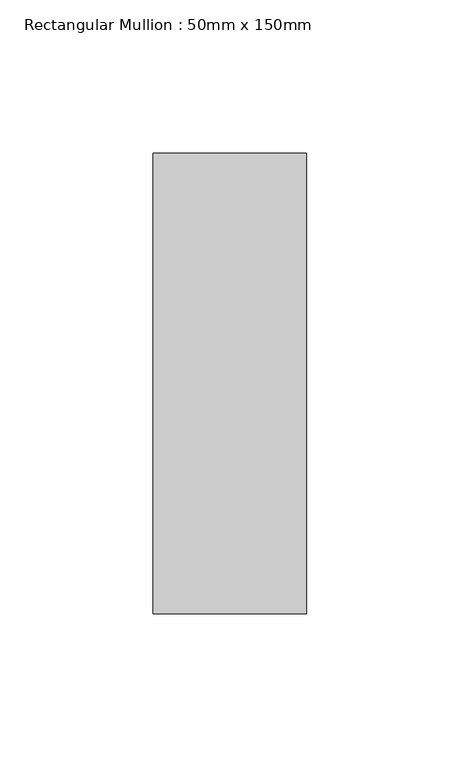
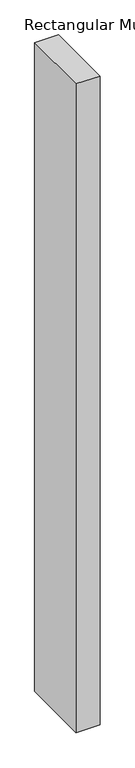
"""IFC4 building model written with IfcOpenShell, lengths in millimetres: member geometry, Rectangular Mullion : 50mm x 150mm."""

from ifc_helpers import new_model, si_unit, frame, origin, place, context, project, spatial, polyline, outline, extrude, source, transform, mapped, element, save


def rectangular_mullion_50mm_x_150mm_f5d81ac7(model_context):
    return source(origin(), model_context, "Body", "SweptSolid", [
        extrude(outline(polyline([(0.0, 75.0), (0.0, -75.0), (-50.0, -75.0), (-50.0, 75.0), (0.0, 75.0)])), frame((0.0, 0.0, -1436.0169252), z_axis=(0.0, 0.0, 1.0), x_axis=(1.0, 0.0, 0.0)), (0.0, 0.0, 1.0), 1436.0169252),
    ])


if __name__ == "__main__":
    model = new_model("IFC4")
    model_context = context("Model", 3, world=origin())
    ifc_project = project(units=[si_unit("LENGTHUNIT", "METRE", prefix="MILLI")], contexts=[model_context])
    site = spatial("IfcSite", under=ifc_project)
    building = spatial("IfcBuilding", under=site)
    placement = place(None, origin())
    rectangular_mullion_50mm_x_150mm_shape = rectangular_mullion_50mm_x_150mm_f5d81ac7(model_context)
    element("IfcMember", 1, ObjectType="Rectangular Mullion : 50mm x 150mm", at=placement, inside=building, context=model_context, shape_type="MappedRepresentation", body=[
        mapped(rectangular_mullion_50mm_x_150mm_shape, transform((0.0, 0.0, 0.0), x_axis=(1.0, 0.0, 0.0), y_axis=(0.0, 1.0, 0.0), z_axis=(0.0, 0.0, 1.0))),
    ])
    save(model, "model.ifc")

# Revit data of these elements
# Type "Rectangular Mullion : 50mm x 150mm"
#   built-in parameter 1007304 = 0.492126 (stored number, unit not read)
#   built-in parameter 1007301 = 0.082021 (stored number, unit not read)
#   built-in parameter 1007300 = 0.082021 (stored number, unit not read)
# Element 1 (IfcMember, "Rectangular Mullion : 50mm x 150mm")
#   Materials on its faces: "Aluminum"
# Materials
#   "Aluminum": class "Metal", colour RGB 244 244 244, transparency 0, Description = "Aluminum 6061", Cost = 0
